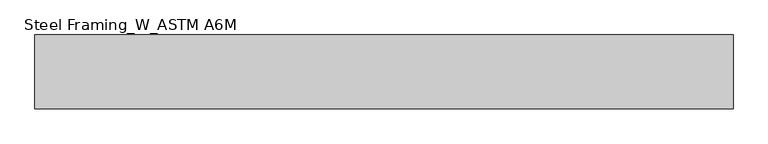
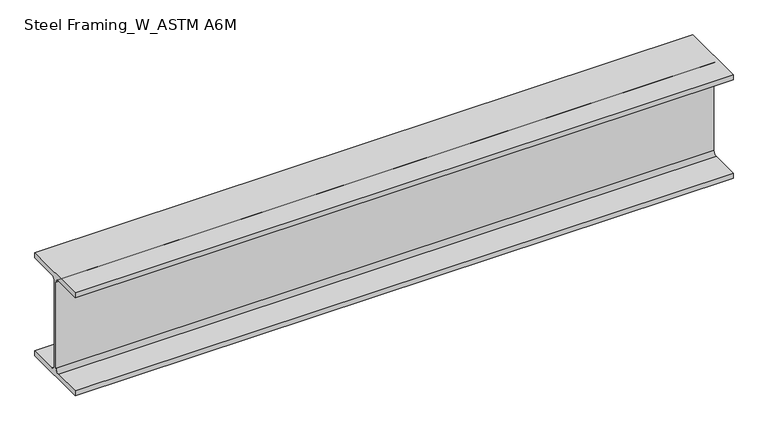
"""IFC4 building model written with IfcOpenShell, lengths in millimetres: beam geometry, Steel Framing_W_ASTM A6M : H_SB_AR_S02_W200x31.3_B6."""

from ifc_helpers import new_model, si_unit, point, frame, frame_2d, origin, place, context, project, spatial, polyline, circle_curve, trimmed, segment, composite_curve, outline, extrude, source, transform, mapped, element, save


def steel_framing_w_astm_a6m_a7324f37(model_context):
    return source(origin(), model_context, "Body", "SweptSolid", [
        extrude(outline(composite_curve([segment(polyline([(67.0, -94.8), (67.0, -105.0), (-67.0, -105.0), (-67.0, -94.8), (-10.775, -94.8)]), True, "CONTINUOUS"), segment(trimmed(circle_curve(frame_2d((-10.775, -87.2)), 7.6), [point((-10.775, -94.8))], [point((-3.175, -87.2))], True, "CARTESIAN"), True, "CONTINUOUS"), segment(polyline([(-3.175, -87.2), (-3.175, 87.2)]), True, "CONTINUOUS"), segment(trimmed(circle_curve(frame_2d((-10.775, 87.2)), 7.6), [point((-3.175, 87.2))], [point((-10.775, 94.8))], True, "CARTESIAN"), True, "CONTINUOUS"), segment(polyline([(-10.775, 94.8), (-67.0, 94.8), (-67.0, 105.0), (67.0, 105.0), (67.0, 94.8), (10.775, 94.8)]), True, "CONTINUOUS"), segment(trimmed(circle_curve(frame_2d((10.775, 87.2)), 7.6), [point((10.775, 94.8))], [point((3.175, 87.2))], True, "CARTESIAN"), True, "CONTINUOUS"), segment(polyline([(3.175, 87.2), (3.175, -87.2)]), True, "CONTINUOUS"), segment(trimmed(circle_curve(frame_2d((10.775, -87.2)), 7.6), [point((3.175, -87.2))], [point((10.775, -94.8))], True, "CARTESIAN"), True, "CONTINUOUS"), segment(polyline([(10.775, -94.8), (67.0, -94.8)]), True, "CONTINUOUS")], self_intersect=False)), frame((-596.3, 0.0, 0.0), z_axis=(1.0, 0.0, 0.0), x_axis=(0.0, 1.0, 0.0)), (0.0, 0.0, 1.0), 1266.6),
    ])


if __name__ == "__main__":
    model = new_model("IFC4")
    model_context = context("Model", 3, world=origin())
    ifc_project = project(units=[si_unit("LENGTHUNIT", "METRE", prefix="MILLI")], contexts=[model_context])
    site = spatial("IfcSite", under=ifc_project)
    building = spatial("IfcBuilding", under=site)
    placement = place(None, origin())
    steel_framing_w_astm_a6m_shape = steel_framing_w_astm_a6m_a7324f37(model_context)
    element("IfcBeam", 1, ObjectType="Steel Framing_W_ASTM A6M : H_SB_AR_S02_W200x31.3_B6", at=placement, inside=building, context=model_context, shape_type="MappedRepresentation", body=[
        mapped(steel_framing_w_astm_a6m_shape, transform((0.0, 0.0, 0.0), x_axis=(1.0, 0.0, 0.0), y_axis=(0.0, 1.0, 0.0), z_axis=(0.0, 0.0, 1.0))),
    ])
    save(model, "model.ifc")

# Revit data of these elements
# Type "Steel Framing_W_ASTM A6M : H_SB_AR_S02_W200x31.3_B6"
#   Type Mark = "B6"
#   Section Name Key = "W8x21"
#   Width = 13.4 cm
#   Web Thickness = 0.635 cm
#   Web Fillet = 0.76 cm
#   Warping Constant = 40800.0 cm⁶
#   Torsional Moment of Inertia = 11.70 cm⁴
#   Section Area = 39.7 cm²
#   Plastic Modulus weak axis = 93.2 cm³
#   Plastic Modulus strong axis = 334.0 cm³
#   Perimeter = 0.93 m²/m
#   Nominal Weight = 31.30 kgf/m
#   Moment of Inertia weak axis = 407.00 cm⁴
#   Moment of Inertia strong axis = 3130.00 cm⁴
#   Height = 21.0 cm
#   Flange Thickness = 1.02 cm
#   Elastic Modulus weak axis = 60.8 cm³
#   Elastic Modulus strong axis = 298.0 cm³
#   Centroid Vertical = 10.5 cm
#   Centroid Horizontal = 6.7 cm
#   Length [instance default] = 1500 mm
#   Structural Material [instance default] = Steel, 45-345
#   Bolt Spacing = 0
#   Assembly Code = ""
# Element 1 (IfcBeam, "Steel Framing_W_ASTM A6M : H_SB_AR_S02_W200x31.3_B6")
#   Materials on its faces: "Steel, 45-345"
# Materials
#   "Steel, 45-345": class "Metal", colour RGB 189 187 185, transparency 0, Description = "Steel 345 MPa", Cost = 0
